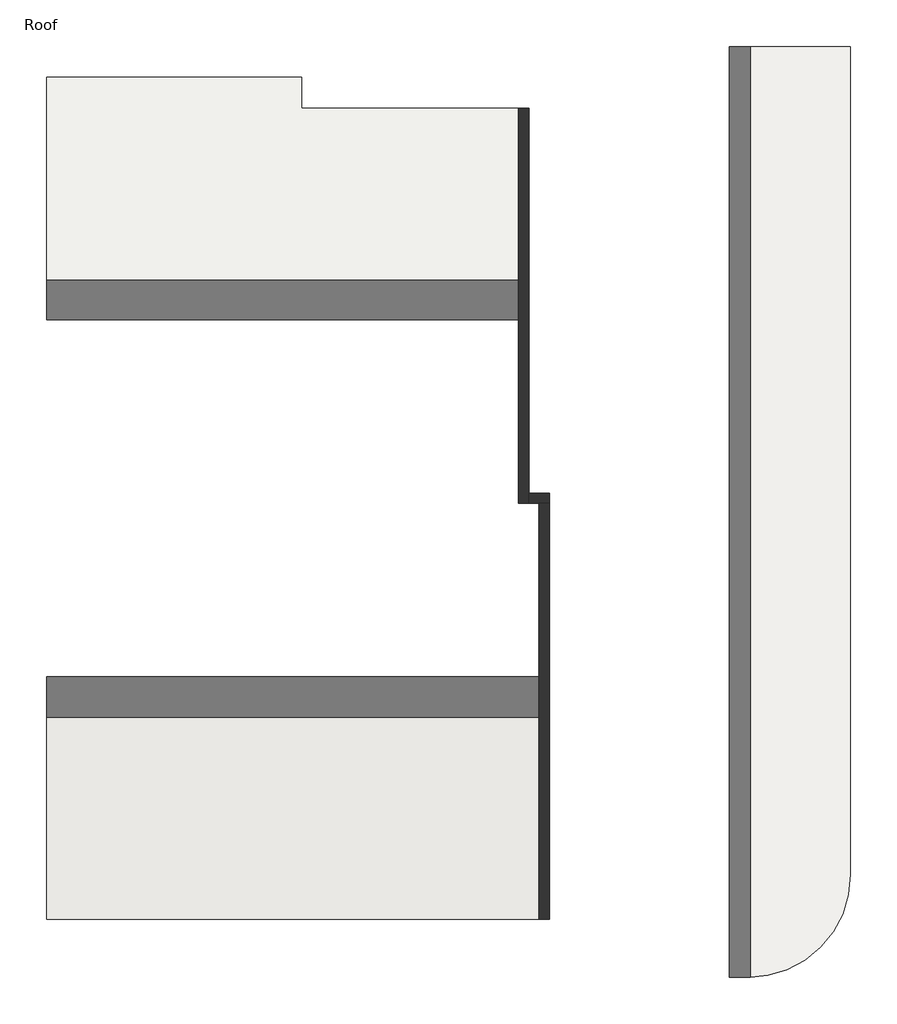
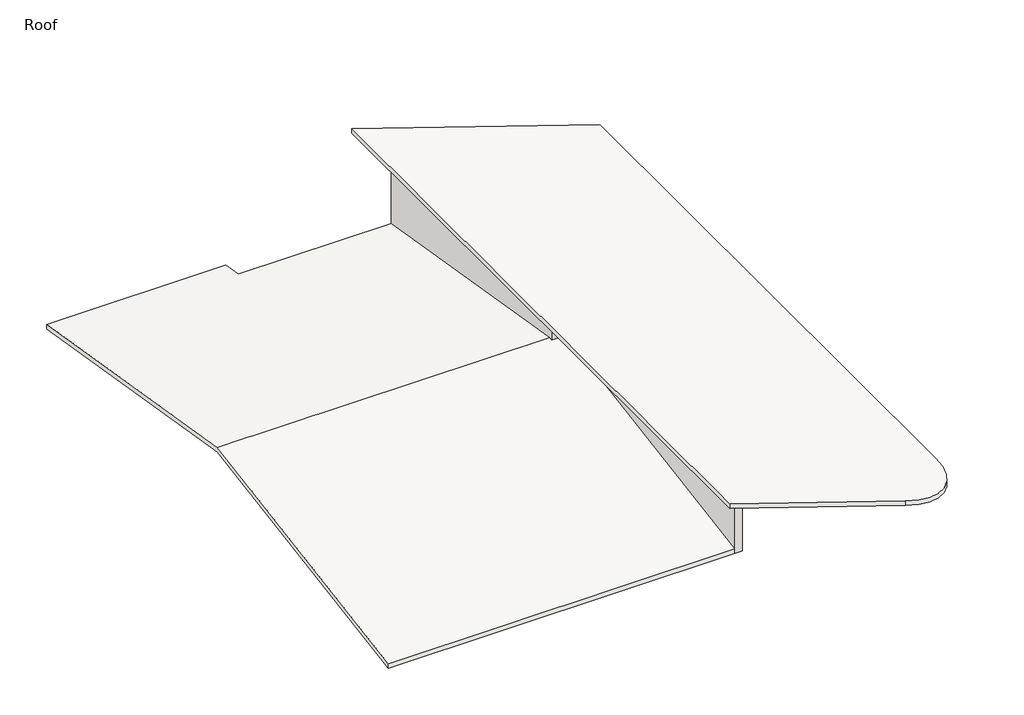
# One storey: 3 walls, 2 roofs.
"""IFC4 building model written with IfcOpenShell, lengths in millimetres."""

from ifc_helpers import new_model, si_unit, frame, origin, place, context, project, spatial, polyline, ellipse_curve, outline, extrude, faceted_brep, element, save
from ifc_brep_helpers import plane_surface, cylinder_surface, advanced_brep

model = new_model("IFC4")

# Units and contexts
model_context = context("Model", 3, world=origin())
ifc_project = project(units=[si_unit("LENGTHUNIT", "METRE", prefix="MILLI")], contexts=[model_context])

# Site, building, storey
site = spatial("IfcSite", under=ifc_project)
building = spatial("IfcBuilding", under=site)
storey = spatial("IfcBuildingStorey", under=building, Name="Roof", Elevation=9144.0)

# Roofs
placement = place(None, origin())
element("IfcRoof", 1, ObjectType="Insulation on Metal Deck - EPDM", at=placement, inside=storey, context=model_context, shape_type="AdvancedBrep", body=[
    advanced_brep(
    [(10561.2601743, 11609.8492079, 12632.2666667), (21026.0601743, 11609.8492079, 9144.0), (21026.0601743, -12977.3507921, 9144.0), (17978.0601743, -16025.3507921, 10160.0), (10561.2601743, -16025.3507921, 12632.2666667), (21026.0601743, 11609.8492079, 9351.4981191), (10561.2601743, 11609.8492079, 12839.7647858), (10561.2601743, -16025.3507921, 12839.7647858), (17978.0601743, -16025.3507921, 10367.4981191), (21026.0601743, -12977.3507921, 9351.4981191)],
    [
        (0, 1),
        (1, 2),
        (2, 3, ellipse_curve(frame((17978.0601743, -12977.3507921, 10160.0), z_axis=(-0.3162277660168387, 0.0, -0.9486832980505137), x_axis=(-0.9486832980505137, 0.0, 0.31622776601683816)), 3212.8741027, 3048.0)),
        (3, 4),
        (4, 0),
        (5, 6),
        (6, 7),
        (7, 8),
        (8, 9, ellipse_curve(frame((17978.0601743, -12977.3507921, 10367.4981191), z_axis=(0.31622776601683866, 0.0, 0.9486832980505137), x_axis=(-0.9486832980505137, 0.0, 0.31622776601683816)), 3212.8741027, 3048.0)),
        (9, 5),
        (1, 5),
        (9, 2),
        (0, 6),
        (4, 7),
        (3, 8),
    ],
    [
        plane_surface(frame((21026.0601743, -12977.3507921, 9144.0), z_axis=(-0.3162277660168387, 0.0, -0.9486832980505137), x_axis=(0.0, 1.0, 0.0))),
        plane_surface(frame((21026.0601743, -12977.3507921, 9351.4981191), z_axis=(0.31622776601683866, 0.0, 0.9486832980505137), x_axis=(0.0, 1.0, 0.0))),
        plane_surface(frame((21026.0601743, -683.7507921, 9144.0), z_axis=(1.0, 0.0, 0.0), x_axis=(0.0, 1.0, 0.0))),
        plane_surface(frame((21026.0601743, 11609.8492079, 0.0), z_axis=(0.0, 1.0, 0.0), x_axis=(-1.0, 0.0, 0.0))),
        plane_surface(frame((10561.2601743, 11609.8492079, 0.0), z_axis=(-1.0, 0.0, 0.0), x_axis=(0.0, -1.0, 0.0))),
        plane_surface(frame((10561.2601743, -16025.3507921, 0.0), z_axis=(0.0, -1.0, 0.0), x_axis=(1.0, 0.0, 0.0))),
        cylinder_surface(frame((17978.0601743, -12977.3507921, 0.0), z_axis=(0.0, 0.0, 1.0), x_axis=(1.0, 0.0, 0.0)), 3048.0),
    ],
    [
        (0, [[1, 2, 3, 4, 5]]),
        (1, [[6, 7, 8, 9, 10]]),
        (2, [[11, -10, 12, -2]]),
        (3, [[-6, -11, -1, 13]]),
        (4, [[-7, -13, -5, 14]]),
        (5, [[-8, -14, -4, 15]]),
        (6, [[-9, -15, -3, -12]]),
    ],
),
])
element("IfcRoof", 2, ObjectType="Insulation on Metal Deck - EPDM", at=placement, inside=storey, context=model_context, shape_type="Brep", body=[
    faceted_brep([(-2849.9398257, -1801.3507921, 11226.8), (-2849.9398257, 10695.4492079, 9144.0), (4719.2601743, 10695.4492079, 9144.0), (4719.2601743, 9781.0492079, 9296.4), (11170.8601743, 9781.0492079, 9296.4), (11170.8601743, -1801.3507921, 11226.8), (11780.4601743, -14298.1507921, 9144.0), (-2849.9398257, -14298.1507921, 9144.0), (11170.8601743, -1953.7507921, 11201.4), (11780.4601743, -1953.7507921, 11201.4), (-2849.9398257, 10695.4492079, 9343.5653007), (-2849.9398257, -1801.3507921, 11426.3653007), (11170.8601743, -1801.3507921, 11426.3653007), (11170.8601743, 9781.0492079, 9495.9653007), (4719.2601743, 9781.0492079, 9495.9653007), (4719.2601743, 10695.4492079, 9343.5653007), (-2849.9398257, -14298.1507921, 9343.5653007), (11780.4601743, -14298.1507921, 9343.5653007), (11780.4601743, -1953.7507921, 11400.9653007), (11170.8601743, -1953.7507921, 11400.9653007)], [[[0, 1, 2, 3, 4, 5]], [[6, 7, 0, 5, 8, 9]], [[10, 11, 12, 13, 14, 15]], [[16, 17, 18, 19, 12, 11]], [[6, 17, 16, 7]], [[1, 10, 15, 2]], [[16, 11, 10, 1, 0, 7]], [[13, 12, 19, 8, 5, 4]], [[15, 14, 3, 2]], [[14, 13, 4, 3]], [[19, 18, 9, 8]], [[18, 17, 6, 9]]]),
])

# Walls
element("IfcWall", 3, ObjectType="Generic - 12\"", at=placement, inside=storey, context=model_context, shape_type="Brep", body=[
    faceted_brep([(11170.8601743, 9781.0492079, 9144.0), (11170.8601743, -1953.7507921, 9144.0), (11170.8601743, -1953.7507921, 12429.0666667), (11170.8601743, 9781.0492079, 12429.0666667), (11475.6601743, 9781.0492079, 9144.0), (11475.6601743, 9781.0492079, 12327.4666667), (11475.6601743, -1648.9507921, 12327.4666667), (11475.6601743, -1953.7507921, 12327.4666667), (11475.6601743, -1953.7507921, 9144.0), (11475.6601743, -1648.9507921, 9144.0)], [[[0, 1, 2, 3]], [[4, 5, 6, 7, 8, 9]], [[1, 0, 4, 9, 8]], [[2, 1, 8, 7]], [[3, 2, 7, 6, 5]], [[0, 3, 5, 4]]]),
])
element("IfcWall", 4, ObjectType="Generic - 12\"", at=placement, inside=storey, context=model_context, shape_type="Brep", body=[
    faceted_brep([(11475.6601743, -1953.7507921, 9144.0), (11780.4601743, -1953.7507921, 9144.0), (12085.2601743, -1953.7507921, 9144.0), (12085.2601743, -1953.7507921, 12124.2666667), (11780.4601743, -1953.7507921, 12225.8666667), (11475.6601743, -1953.7507921, 12327.4666667), (11475.6601743, -1648.9507921, 9144.0), (11475.6601743, -1648.9507921, 12327.4666667), (12085.2601743, -1648.9507921, 12124.2666667), (12085.2601743, -1648.9507921, 9144.0)], [[[0, 1, 2, 3, 4, 5]], [[6, 7, 8, 9]], [[2, 1, 0, 6, 9]], [[0, 5, 7, 6]], [[3, 2, 9, 8]], [[5, 4, 3, 8, 7]]]),
])
element("IfcWall", 5, ObjectType="Generic - 12\"", at=placement, inside=storey, context=model_context, shape_type="SweptSolid", body=[
    extrude(outline(polyline([(9144.0, 12085.2601743), (12124.2666667, 12085.2601743), (12225.8666667, 11780.4601743), (9144.0, 11780.4601743), (9144.0, 12085.2601743)])), frame((0.0, -14298.1507921, 0.0), z_axis=(0.0, 1.0, 0.0), x_axis=(0.0, 0.0, 1.0)), (0.0, 0.0, 1.0), 12344.4),
])

save(model, "model.ifc")

# Revit data of these elements
# Project information
#   Project Issue Date = "Issue Date"
#   Project Status = "Project Status"
#   Client Name = "Owner"
#   Project Address = "Enter address here"
#   Project Name = "Project Name"
#   Project Number = "Project Number"
# Grids (mm)
#   "1": line (-17480.34, 14427.416) -> (-17480.34, -18533.688)
#   "2": line (-10165.14, 14427.416) -> (-10165.14, -18533.688)
#   "3": line (-2849.94, 14427.416) -> (-2849.94, -18533.688)
#   "4": line (4465.26, 14427.416) -> (4465.26, -18533.688)
#   "5": line (11780.46, 14427.416) -> (11780.46, -18533.688)
#   "6": line (19095.66, 14427.416) -> (19095.66, -18533.688)
#   "A": line (-21295.126, -13993.351) -> (21386.076, -13993.351)
#   "B": line (-21295.126, -5458.951) -> (21386.076, -5458.951)
#   "C": line (-21295.126, 3075.449) -> (21386.076, 3075.449)
#   "D": line (-21295.126, 10390.649) -> (21386.076, 10390.649)
# Type "Insulation on Metal Deck - EPDM"
#   Assembly Code = "B1020"
#   Layers, outside or top first: 0' - 0 1/4" "Roofing, EPDM Membrane" (function 4); 0' - 3" "Rigid insulation" (function 3); 0' - 3" "Concrete, Cast-in-Place gray" (function 1); 0' - 1 1/2" "Metal Deck" (function 1)
# Type "Generic - 12\""
#   Assembly Code = "B2010"
#   Layers, outside or top first: 1' - 0" no material (function 1)
# Element 1 (IfcRoof, "Insulation on Metal Deck - EPDM")
#   built-in parameter 1001705 = 42.1252 (stored number, unit not read)
#   built-in parameter 1001710 = 33615
#   Phase Created = New Construction
#   Materials on its faces: "Metal Deck", "Roofing, EPDM Membrane"
# Element 2 (IfcRoof, "Insulation on Metal Deck - EPDM")
#   built-in parameter 1001705 = 37.4881 (stored number, unit not read)
#   built-in parameter 1001710 = 33615
#   Phase Created = New Construction
#   Materials on its faces: "Metal Deck", "Roofing, EPDM Membrane"
# Elements 3, 4, 5 (IfcWall, "Generic - 12\"")
#   Top Offset = 0' - 0"
#   Base Offset = 0' - 0"
#   wall height = 3' - 0"
#   Phase Created = New Construction
#   Base Constraint = Roof
#   Top Constraint = Parapet
#   Materials on its faces: "Default Wall"
# Materials
#   "Roofing, EPDM Membrane": class "Generic", colour RGB 127 127 127, transparency 0, Description = "EPDM roof membrane", Cost = 0
#   "Rigid insulation": class "Generic", colour RGB 127 127 127, transparency 0, Description = "Rigid foam insulation board", Cost = 0
#   "Concrete, Cast-in-Place gray": class "Concrete", colour RGB 192 192 192, transparency 0, Description = "Cast-in-place concrete", Cost = 0
#   "Metal Deck": class "Metal", colour RGB 199 199 199, transparency 0, Description = "Steel, mill finish", Cost = 0
#   "Default Wall": class "Miscellaneous", colour RGB 127 127 127, transparency 0
